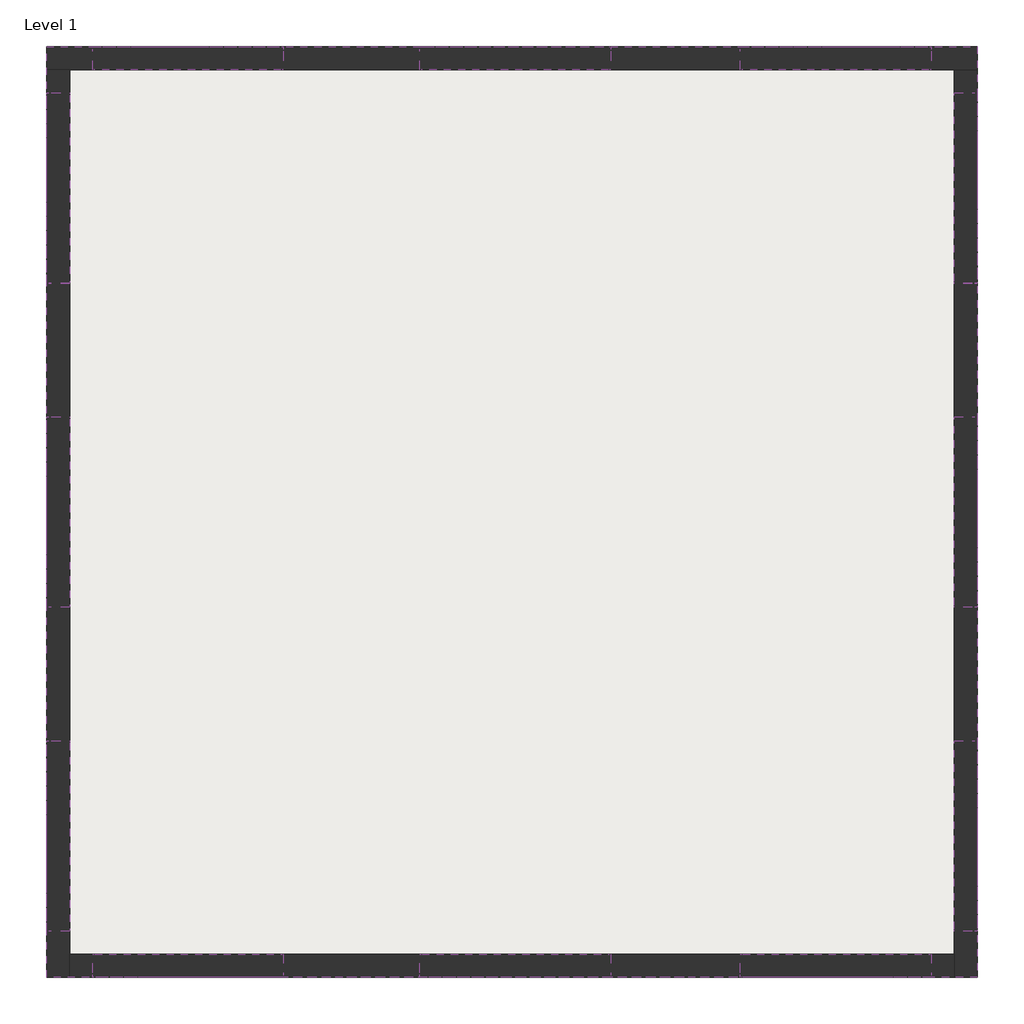
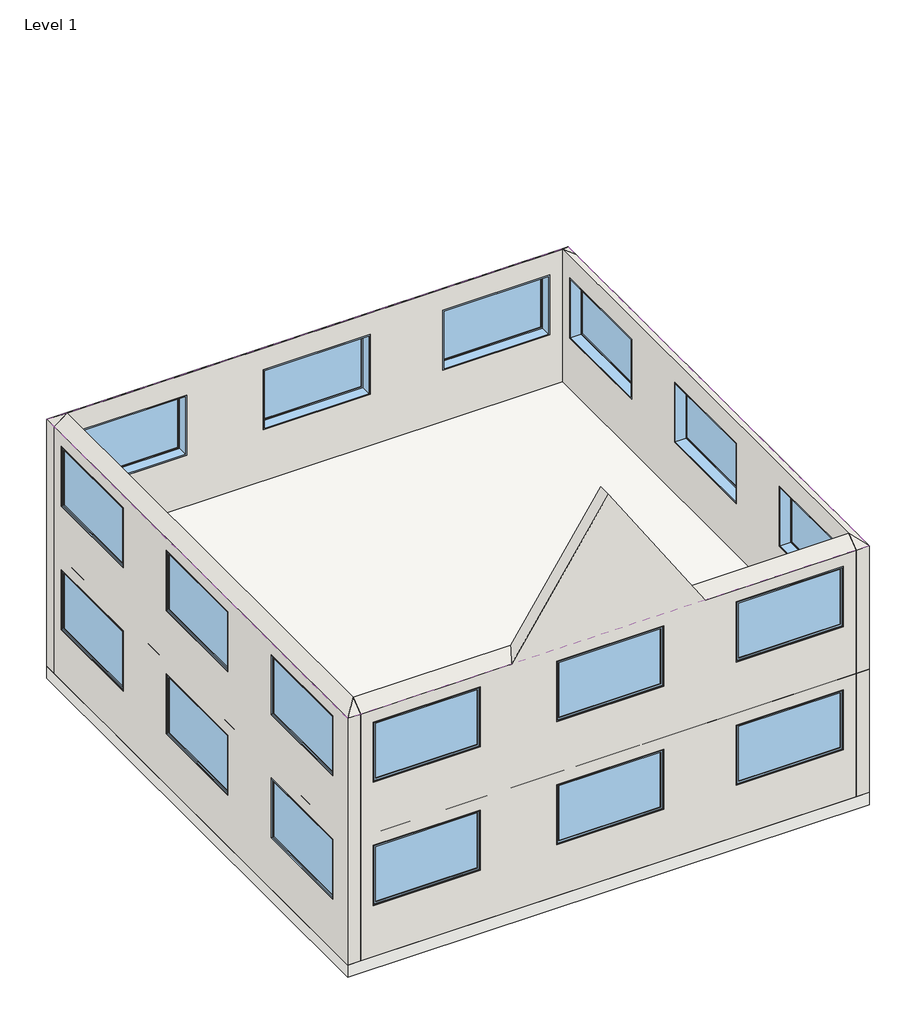
# One storey: 24 windows, 4 walls, 2 slabs, 1 roof.
"""IFC4 building model written with IfcOpenShell, lengths in millimetres."""

import ifcopenshell
import ifcopenshell.guid

model = None  # the IFC model being written
_history = None  # IfcOwnerHistory: only IFC2X3 demands one
_inside = {}  # id of a spatial element -> (the spatial element, [elements in it])
_under = {}  # id of a project, library or spatial element -> (it, [spatial elements below it])
_declared = {}  # id of a project -> (the project, [libraries it declares])
_typed = {}  # id of a type object -> (the type object, [elements of that type])
_made_of = {}  # id of a material, layer set ... -> (it, [elements and type objects made of it])


def new_model(schema):
    """Start an empty IFC model of exactly this schema.

    Asked for "IFC4X3", IfcOpenShell would pick the latest addendum, in which some entities
    have other attributes; the version numbers below select the first issue.
    IFC2X3 requires an IfcOwnerHistory on every rooted entity: one is made here for all.
    """
    global model, _history
    if schema == "IFC4X3":
        model = ifcopenshell.file(schema_version=(4, 3, 0, 0))
    else:
        model = ifcopenshell.file(schema=schema)
    _inside.clear()
    _under.clear()
    _declared.clear()
    _typed.clear()
    _made_of.clear()
    _history = None
    if model.schema == "IFC2X3":
        org = make("IfcOrganization", Name="unknown")
        user = make(
            "IfcPersonAndOrganization",
            ThePerson=make("IfcPerson", FamilyName="unknown"),
            TheOrganization=org,
        )
        app = make(
            "IfcApplication",
            ApplicationDeveloper=org,
            Version="unknown",
            ApplicationFullName="unknown",
            ApplicationIdentifier="unknown",
        )
        _history = make(
            "IfcOwnerHistory",
            OwningUser=user,
            OwningApplication=app,
            ChangeAction="ADDED",
            CreationDate=0,
        )
    return model


def make(cls, **values):
    """One entity of the class cls with the attributes given. An attribute that is None is left unset."""
    return model.create_entity(
        cls, **{name: value for name, value in values.items() if value is not None}
    )


def rooted(cls, **values):
    """An entity with a GlobalId (a new one), such as an element, a storey or a relation."""
    return make(cls, GlobalId=ifcopenshell.guid.new(), OwnerHistory=_history, **values)


def si_unit(unit_type, name, prefix=None):
    """IfcSIUnit, for example si_unit("LENGTHUNIT", "METRE", prefix="MILLI")."""
    return make("IfcSIUnit", UnitType=unit_type, Prefix=prefix, Name=name)


def assignment(units):
    """IfcUnitAssignment: the units of a project."""
    return None if units is None else make("IfcUnitAssignment", Units=units)


def point(xyz):
    """IfcCartesianPoint."""
    return None if xyz is None else make("IfcCartesianPoint", Coordinates=xyz)


def direction(xyz):
    """IfcDirection."""
    return None if xyz is None else make("IfcDirection", DirectionRatios=xyz)


def frame(location, z_axis=None, x_axis=None):
    """IfcAxis2Placement3D, a coordinate frame: its origin and axes. An axis left out is left unset."""
    return make(
        "IfcAxis2Placement3D",
        Location=point(location),
        Axis=direction(z_axis),
        RefDirection=direction(x_axis),
    )


def origin():
    """The frame at (0, 0, 0) with its axes left unset."""
    return frame((0.0, 0.0, 0.0))


def place(relative_to, where):
    """IfcLocalPlacement: puts the frame where relative to a parent placement (None: the world)."""
    return make(
        "IfcLocalPlacement", PlacementRelTo=relative_to, RelativePlacement=where
    )


def context(
    kind, dimensions, precision=None, world=None, true_north=None, identifier=None
):
    """IfcGeometricRepresentationContext, for example the 3D "Model" context."""
    return make(
        "IfcGeometricRepresentationContext",
        ContextIdentifier=identifier,
        ContextType=kind,
        CoordinateSpaceDimension=dimensions,
        Precision=precision,
        WorldCoordinateSystem=world,
        TrueNorth=true_north,
    )


def project(units=None, contexts=None):
    """IfcProject with its units and contexts."""
    return rooted(
        "IfcProject",
        Name="project",
        RepresentationContexts=contexts,
        UnitsInContext=assignment(units),
    )


def spatial(cls, under=None, at=None, **own):
    """A site, building, storey or space (cls), placed at a placement, below another one or the project."""
    s = rooted(cls, ObjectPlacement=at, **own)
    if under is not None:
        _under.setdefault(under.id(), (under, []))[1].append(s)
    return s


def polyline(points):
    """IfcPolyline through the points."""
    return make("IfcPolyline", Points=[point(p) for p in points])


def outline(outer, holes=None, kind="AREA"):
    """IfcArbitraryClosedProfileDef: a profile drawn as a closed curve; with holes, ...WithVoids."""
    if holes is None:
        return make("IfcArbitraryClosedProfileDef", ProfileType=kind, OuterCurve=outer)
    return make(
        "IfcArbitraryProfileDefWithVoids",
        ProfileType=kind,
        OuterCurve=outer,
        InnerCurves=holes,
    )


def extrude(swept, where, along, depth):
    """IfcExtrudedAreaSolid: the profile swept, set in the frame where, extruded along a direction by depth."""
    return make(
        "IfcExtrudedAreaSolid",
        SweptArea=swept,
        Position=where,
        ExtrudedDirection=direction(along),
        Depth=depth,
    )


def faces_of(points, faces, orient=None, outer=None):
    """IfcFace entities. A face is a list of loops; a loop is a list of indices into points, from 0.

    orient and outer hold one flag for each loop. By default every Orientation is true, the
    first loop of a face is its IfcFaceOuterBound and the others are IfcFaceBound.
    """
    made = []
    for i, loops in enumerate(faces):
        bounds = []
        for j, loop in enumerate(loops):
            is_outer = j == 0 if outer is None else outer[i][j]
            bounds.append(
                make(
                    "IfcFaceOuterBound" if is_outer else "IfcFaceBound",
                    Bound=make("IfcPolyLoop", Polygon=[points[k] for k in loop]),
                    Orientation=True if orient is None else orient[i][j],
                )
            )
        made.append(make("IfcFace", Bounds=bounds))
    return made


def faceted_brep(points, faces, orient=None, outer=None, voids=None):
    """IfcFacetedBrep: a solid bounded by flat faces; with voids (closed shells), ...WithVoids."""
    shared = [point(p) for p in points]
    hull = make("IfcClosedShell", CfsFaces=faces_of(shared, faces, orient, outer))
    if voids is None:
        return make("IfcFacetedBrep", Outer=hull)
    return make(
        "IfcFacetedBrepWithVoids",
        Outer=hull,
        Voids=[
            make(cls, CfsFaces=faces_of(shared, fs, o, b)) for cls, fs, o, b in voids
        ],
    )


def shape(context_of_items, identifier, shape_type, items):
    """IfcShapeRepresentation: the items that make up one representation, for example the "Body"."""
    return make(
        "IfcShapeRepresentation",
        ContextOfItems=context_of_items,
        RepresentationIdentifier=identifier,
        RepresentationType=shape_type,
        Items=items,
    )


def source(mapping_origin, context_of_items, identifier, shape_type, items):
    """IfcRepresentationMap: a shape defined once, which mapped items show again and again."""
    return make(
        "IfcRepresentationMap",
        MappingOrigin=mapping_origin,
        MappedRepresentation=shape(context_of_items, identifier, shape_type, items),
    )


def transform(
    local_origin,
    x_axis=None,
    y_axis=None,
    z_axis=None,
    scale=None,
    scale2=None,
    scale3=None,
    uniform=True,
):
    """IfcCartesianTransformationOperator3D, or its non-uniform kind. x_axis, y_axis, z_axis: its Axis1, 2, 3."""
    if uniform:
        return make(
            "IfcCartesianTransformationOperator3D",
            Axis1=direction(x_axis),
            Axis2=direction(y_axis),
            LocalOrigin=point(local_origin),
            Scale=scale,
            Axis3=direction(z_axis),
        )
    return make(
        "IfcCartesianTransformationOperator3DnonUniform",
        Axis1=direction(x_axis),
        Axis2=direction(y_axis),
        LocalOrigin=point(local_origin),
        Scale=scale,
        Axis3=direction(z_axis),
        Scale2=scale2,
        Scale3=scale3,
    )


def mapped(mapping_source, mapping_target):
    """IfcMappedItem: shows the shape of a source again, moved by a transform."""
    return make(
        "IfcMappedItem", MappingSource=mapping_source, MappingTarget=mapping_target
    )


def made_of(thing, what):
    """Note that an element or type object is made of a material, layer set ...; save() writes the relation."""
    if what is not None:
        _made_of.setdefault(what.id(), (what, []))[1].append(thing)
    return thing


def element(
    cls,
    number,
    at=None,
    inside=None,
    cuts=None,
    type_object=None,
    material=None,
    context=None,
    identifier="Body",
    shape_type=None,
    held_by="IfcProductDefinitionShape",
    body=None,
    shapes=None,
    **own,
):
    """One element of the class cls, such as IfcWall. Its Tag is "e" and its number.

    at: its placement. inside: the storey or other place that contains it. cuts: it is an
    opening in that element (IfcRelVoidsElement). A single representation is given by context,
    identifier, shape_type and body (its items); several are given by shapes. held_by: the class
    of the entity that holds the representations. save() writes the other relations.
    """
    e = rooted(cls, Tag="e%d" % number, ObjectPlacement=at, **own)
    if body is not None:
        shapes = [shape(context, identifier, shape_type, body)]
    if shapes is not None:
        e.Representation = make(held_by, Representations=shapes)
    if inside is not None:
        _inside.setdefault(inside.id(), (inside, []))[1].append(e)
    if cuts is not None:
        rooted(
            "IfcRelVoidsElement", RelatingBuildingElement=cuts, RelatedOpeningElement=e
        )
    if type_object is not None:
        _typed.setdefault(type_object.id(), (type_object, []))[1].append(e)
    return made_of(e, material)


def aggregate(whole, parts):
    """IfcRelAggregates: a whole, such as a stair, and the parts it consists of."""
    return rooted("IfcRelAggregates", RelatingObject=whole, RelatedObjects=parts)


def save(model, path):
    """Write the relations noted so far, then the file.

    IfcRelAggregates (storeys below a building ...), IfcRelContainedInSpatialStructure (elements
    in a storey), IfcRelDefinesByType, IfcRelAssociatesMaterial and IfcRelDeclares: one each for
    every whole, place, type object, material and project.
    """
    for whole, parts in _under.values():
        aggregate(whole, parts)
    for where, things in _inside.values():
        rooted(
            "IfcRelContainedInSpatialStructure",
            RelatedElements=things,
            RelatingStructure=where,
        )
    for kind, things in _typed.values():
        rooted("IfcRelDefinesByType", RelatedObjects=things, RelatingType=kind)
    for what, things in _made_of.values():
        rooted("IfcRelAssociatesMaterial", RelatedObjects=things, RelatingMaterial=what)
    for by, libraries in _declared.values():
        rooted("IfcRelDeclares", RelatingContext=by, RelatedDefinitions=libraries)
    model.write(path)


def m_fixed_2500_x_1486mm_baf7df51(model_context):
    return source(origin(), model_context, "Body", "SweptSolid", [
        extrude(outline(polyline([(-1187.0, 130.4), (1187.0, 130.4), (1187.0, 118.4), (-1187.0, 118.4), (-1187.0, 130.4)])), frame((0.0, 0.0, 978.0), z_axis=(0.0, 0.0, 1.0), x_axis=(1.0, 0.0, 0.0)), (0.0, 0.0, 1.0), 1360.5),
        extrude(outline(polyline([(2382.5, -1231.0), (934.0, -1231.0), (934.0, 1231.0), (2382.5, 1231.0), (2382.5, -1231.0)]), holes=[polyline([(2338.5, -1187.0), (2338.5, 1187.0), (978.0, 1187.0), (978.0, -1187.0), (2338.5, -1187.0)])]), frame((0.0, 102.4, 0.0), z_axis=(0.0, 1.0, 0.0), x_axis=(0.0, 0.0, 1.0)), (0.0, 0.0, 1.0), 44.0),
        extrude(outline(polyline([(2401.5, -1250.0), (915.0, -1250.0), (915.0, 1250.0), (2401.5, 1250.0), (2401.5, -1250.0)]), holes=[polyline([(2382.5, -1231.0), (2382.5, 1231.0), (934.0, 1231.0), (934.0, -1231.0), (2382.5, -1231.0)])]), frame((0.0, 102.4, 0.0), z_axis=(0.0, 1.0, 0.0), x_axis=(0.0, 0.0, 1.0)), (0.0, 0.0, 1.0), 63.0),
        extrude(outline(polyline([(2401.5, -1250.0), (915.0, -1250.0), (915.0, 1250.0), (2401.5, 1250.0), (2401.5, -1250.0)]), holes=[polyline([(2369.5, -1218.0), (2369.5, 1218.0), (947.0, 1218.0), (947.0, -1218.0), (2369.5, -1218.0)])]), frame((0.0, -139.4, 0.0), z_axis=(0.0, 1.0, 0.0), x_axis=(0.0, 0.0, 1.0)), (0.0, 0.0, 1.0), 241.8),
    ])


def m_fixed_2500_x_1486mm_49bc14c1(model_context):
    return source(origin(), model_context, "Body", "SweptSolid", [
        extrude(outline(polyline([(-1187.0, -130.4), (-1187.0, -118.4), (1187.0, -118.4), (1187.0, -130.4), (-1187.0, -130.4)])), frame((0.0, 0.0, 978.0), z_axis=(0.0, 0.0, 1.0), x_axis=(1.0, 0.0, 0.0)), (0.0, 0.0, 1.0), 1360.5),
        extrude(outline(polyline([(2382.5, -1231.0), (934.0, -1231.0), (934.0, 1231.0), (2382.5, 1231.0), (2382.5, -1231.0)]), holes=[polyline([(2338.5, -1187.0), (2338.5, 1187.0), (978.0, 1187.0), (978.0, -1187.0), (2338.5, -1187.0)])]), frame((0.0, -146.4, 0.0), z_axis=(0.0, 1.0, 0.0), x_axis=(0.0, 0.0, 1.0)), (0.0, 0.0, 1.0), 44.0),
        extrude(outline(polyline([(2401.5, -1250.0), (915.0, -1250.0), (915.0, 1250.0), (2401.5, 1250.0), (2401.5, -1250.0)]), holes=[polyline([(2382.5, -1231.0), (2382.5, 1231.0), (934.0, 1231.0), (934.0, -1231.0), (2382.5, -1231.0)])]), frame((0.0, -165.4, 0.0), z_axis=(0.0, 1.0, 0.0), x_axis=(0.0, 0.0, 1.0)), (0.0, 0.0, 1.0), 63.0),
        extrude(outline(polyline([(2401.5, -1250.0), (915.0, -1250.0), (915.0, 1250.0), (2401.5, 1250.0), (2401.5, -1250.0)]), holes=[polyline([(2369.5, -1218.0), (2369.5, 1218.0), (947.0, 1218.0), (947.0, -1218.0), (2369.5, -1218.0)])]), frame((0.0, -102.4, 0.0), z_axis=(0.0, 1.0, 0.0), x_axis=(0.0, 0.0, 1.0)), (0.0, 0.0, 1.0), 241.8),
    ])


model = new_model("IFC4")

# Units and contexts
model_context = context("Model", 3, world=origin())
ifc_project = project(units=[si_unit("LENGTHUNIT", "METRE", prefix="MILLI")], contexts=[model_context])

# Site, building, storey
site = spatial("IfcSite", under=ifc_project)
building = spatial("IfcBuilding", under=site)
storey = spatial("IfcBuildingStorey", under=building, Name="Level 1", Elevation=0.0)

# Roof
placement = place(None, origin())
element("IfcRoof", 1, ObjectType="Generic Roof - 300mm", at=placement, inside=storey, context=model_context, shape_type="Brep", body=[
    faceted_brep([(21465.644102, 9062.7173115, 6096.0), (15369.644102, 2966.7173115, 10668.0170156), (9273.644102, 9062.7173115, 6096.0), (9273.644102, -3129.2826885, 6096.0), (13109.1679245, -3129.2826885, 6096.0), (12998.044102, -3129.2826885, 6096.0), (21465.644102, -3129.2826885, 6096.0), (17741.244102, -3129.2826885, 6096.0), (17630.1202795, -3129.2826885, 6096.0), (15369.644102, 1410.2073073, 9500.6301678), (15369.644102, -3129.2826885, 9500.6301678), (21465.644102, 9062.7173115, 6471.0005024), (9273.644102, 9062.7173115, 6471.0005024), (15369.644102, 2966.7173115, 11043.0175181), (9273.644102, -3129.2826885, 6471.0005024), (12998.044102, -3129.2826885, 6471.0005024), (15369.644102, 1633.366253, 10043.0005024), (17741.244102, -3129.2826885, 6471.0005024), (21465.644102, -3129.2826885, 6471.0005024), (15369.644102, -3129.2826885, 10043.0005024)], [[[0, 1, 2]], [[2, 1, 3]], [[4, 5, 3, 1, 6, 7, 8, 9]], [[6, 1, 0]], [[4, 9, 10]], [[8, 10, 9]], [[11, 12, 13]], [[12, 14, 13]], [[15, 16, 17, 18, 13, 14]], [[18, 11, 13]], [[15, 19, 16]], [[17, 16, 19]], [[6, 18, 17, 7]], [[0, 11, 18, 6]], [[2, 12, 11, 0]], [[3, 14, 12, 2]], [[5, 15, 14, 3]], [[17, 19, 15, 5, 4, 10, 8, 7]]]),
])

# Slabs
element("IfcSlab", 2, ObjectType="Generic Floor - 304.8mm", at=placement, inside=storey, context=model_context, shape_type="Brep", body=[
    faceted_brep([(21465.644102, 9062.7173115, -304.8), (21465.644102, -3129.2826885, -304.8), (9273.644102, -3129.2826885, -304.8), (9273.644102, 9062.7173115, -304.8), (21465.644102, 9062.7173115, 0.0), (9273.644102, 9062.7173115, 0.0), (9273.644102, -3129.2826885, 0.0), (9578.444102, -3129.2826885, 0.0), (21160.844102, -3129.2826885, 0.0), (21465.644102, -3129.2826885, 0.0), (21465.644102, 8757.9173115, 0.0)], [[[0, 1, 2, 3]], [[4, 5, 6, 7, 8, 9, 10]], [[1, 0, 4, 10, 9]], [[2, 1, 9, 8, 7, 6]], [[3, 2, 6, 5]], [[0, 3, 5, 4]]]),
])
element("IfcSlab", 3, ObjectType="Generic Floor - 304.8mm", at=placement, inside=storey, context=model_context, shape_type="SweptSolid", body=[
    extrude(outline(polyline([(21465.644102, 9062.7173115), (21465.644102, -3129.2826885), (9273.644102, -3129.2826885), (9273.644102, 9062.7173115), (21465.644102, 9062.7173115)])), frame((0.0, 0.0, 2743.2), z_axis=(0.0, 0.0, 1.0), x_axis=(1.0, 0.0, 0.0)), (0.0, 0.0, 1.0), 304.8),
])

# Walls
element("IfcWall", 4, ObjectType="Generic - 304.8mm", at=placement, inside=storey, context=model_context, shape_type="Brep", body=[
    faceted_brep([(9273.644102, 8757.9173115, 0.0), (9578.444102, 8757.9173115, 0.0), (21160.844102, 8757.9173115, 0.0), (21465.644102, 8757.9173115, 0.0), (21465.644102, 8757.9173115, 6096.0), (21160.844102, 8757.9173115, 6324.6008508), (9578.444102, 8757.9173115, 6324.6008508), (9273.644102, 8757.9173115, 6096.0), (14163.244102, 8757.9173115, 4309.5), (14163.244102, 8757.9173115, 5796.0), (16663.244102, 8757.9173115, 5796.0), (16663.244102, 8757.9173115, 4309.5), (9876.044102, 8757.9173115, 4309.5), (9876.044102, 8757.9173115, 5796.0), (12376.044102, 8757.9173115, 5796.0), (12376.044102, 8757.9173115, 4309.5), (18363.244102, 8757.9173115, 4309.5), (18363.244102, 8757.9173115, 5796.0), (20863.244102, 8757.9173115, 5796.0), (20863.244102, 8757.9173115, 4309.5), (18363.244102, 8757.9173115, 1261.5), (18363.244102, 8757.9173115, 2748.0), (20863.244102, 8757.9173115, 2748.0), (20863.244102, 8757.9173115, 1261.5), (9876.044102, 8757.9173115, 1261.5), (9876.044102, 8757.9173115, 2748.0), (12376.044102, 8757.9173115, 2748.0), (12376.044102, 8757.9173115, 1261.5), (14163.244102, 8757.9173115, 1261.5), (14163.244102, 8757.9173115, 2748.0), (16663.244102, 8757.9173115, 2748.0), (16663.244102, 8757.9173115, 1261.5), (9273.644102, 9062.7173115, 0.0), (9273.644102, 9062.7173115, 6096.0), (21465.644102, 9062.7173115, 6096.0), (21465.644102, 9062.7173115, 0.0), (14163.244102, 9062.7173115, 4309.5), (16663.244102, 9062.7173115, 4309.5), (16663.244102, 9062.7173115, 5796.0), (14163.244102, 9062.7173115, 5796.0), (9876.044102, 9062.7173115, 4309.5), (12376.044102, 9062.7173115, 4309.5), (12376.044102, 9062.7173115, 5796.0), (9876.044102, 9062.7173115, 5796.0), (18363.244102, 9062.7173115, 4309.5), (20863.244102, 9062.7173115, 4309.5), (20863.244102, 9062.7173115, 5796.0), (18363.244102, 9062.7173115, 5796.0), (18363.244102, 9062.7173115, 1261.5), (20863.244102, 9062.7173115, 1261.5), (20863.244102, 9062.7173115, 2748.0), (18363.244102, 9062.7173115, 2748.0), (9876.044102, 9062.7173115, 1261.5), (12376.044102, 9062.7173115, 1261.5), (12376.044102, 9062.7173115, 2748.0), (9876.044102, 9062.7173115, 2748.0), (14163.244102, 9062.7173115, 1261.5), (16663.244102, 9062.7173115, 1261.5), (16663.244102, 9062.7173115, 2748.0), (14163.244102, 9062.7173115, 2748.0)], [[[0, 1, 2, 3, 4, 5, 6, 7], [8, 9, 10, 11], [12, 13, 14, 15], [16, 17, 18, 19], [20, 21, 22, 23], [24, 25, 26, 27], [28, 29, 30, 31]], [[32, 33, 34, 35], [36, 37, 38, 39], [40, 41, 42, 43], [44, 45, 46, 47], [48, 49, 50, 51], [52, 53, 54, 55], [56, 57, 58, 59]], [[3, 2, 1, 0, 32, 35]], [[4, 3, 35, 34]], [[0, 7, 33, 32]], [[9, 8, 36, 39]], [[10, 9, 39, 38]], [[11, 10, 38, 37]], [[8, 11, 37, 36]], [[13, 12, 40, 43]], [[14, 13, 43, 42]], [[15, 14, 42, 41]], [[12, 15, 41, 40]], [[17, 16, 44, 47]], [[18, 17, 47, 46]], [[19, 18, 46, 45]], [[16, 19, 45, 44]], [[21, 20, 48, 51]], [[22, 21, 51, 50]], [[23, 22, 50, 49]], [[20, 23, 49, 48]], [[25, 24, 52, 55]], [[26, 25, 55, 54]], [[27, 26, 54, 53]], [[24, 27, 53, 52]], [[29, 28, 56, 59]], [[30, 29, 59, 58]], [[31, 30, 58, 57]], [[28, 31, 57, 56]], [[7, 6, 33]], [[6, 5, 34, 33]], [[5, 4, 34]]]),
])
element("IfcWall", 5, ObjectType="Generic - 304.8mm", at=placement, inside=storey, context=model_context, shape_type="Brep", body=[
    faceted_brep([(21160.844102, 8757.9173115, 0.0), (21160.844102, -2824.4826885, 0.0), (21160.844102, -3129.2826885, 0.0), (21160.844102, -3129.2826885, 6096.0), (21160.844102, -2824.4826885, 6324.6008508), (21160.844102, 8757.9173115, 6324.6008508), (21160.844102, -26.8826885, 4309.5), (21160.844102, -26.8826885, 5796.0), (21160.844102, -2526.8826885, 5796.0), (21160.844102, -2526.8826885, 4309.5), (21160.844102, 8460.3173115, 4309.5), (21160.844102, 8460.3173115, 5796.0), (21160.844102, 5960.3173115, 5796.0), (21160.844102, 5960.3173115, 4309.5), (21160.844102, 4216.7173115, 4309.5), (21160.844102, 4216.7173115, 5796.0), (21160.844102, 1716.7173115, 5796.0), (21160.844102, 1716.7173115, 4309.5), (21160.844102, 4216.7173115, 1261.5), (21160.844102, 4216.7173115, 2748.0), (21160.844102, 1716.7173115, 2748.0), (21160.844102, 1716.7173115, 1261.5), (21160.844102, 8460.3173115, 1261.5), (21160.844102, 8460.3173115, 2748.0), (21160.844102, 5960.3173115, 2748.0), (21160.844102, 5960.3173115, 1261.5), (21160.844102, -26.8826885, 1261.5), (21160.844102, -26.8826885, 2748.0), (21160.844102, -2526.8826885, 2748.0), (21160.844102, -2526.8826885, 1261.5), (21465.644102, 8757.9173115, 0.0), (21465.644102, 8757.9173115, 6096.0), (21465.644102, -3129.2826885, 6096.0), (21465.644102, -3129.2826885, 0.0), (21465.644102, -26.8826885, 4309.5), (21465.644102, -2526.8826885, 4309.5), (21465.644102, -2526.8826885, 5796.0), (21465.644102, -26.8826885, 5796.0), (21465.644102, 8460.3173115, 4309.5), (21465.644102, 5960.3173115, 4309.5), (21465.644102, 5960.3173115, 5796.0), (21465.644102, 8460.3173115, 5796.0), (21465.644102, 4216.7173115, 4309.5), (21465.644102, 1716.7173115, 4309.5), (21465.644102, 1716.7173115, 5796.0), (21465.644102, 4216.7173115, 5796.0), (21465.644102, 4216.7173115, 1261.5), (21465.644102, 1716.7173115, 1261.5), (21465.644102, 1716.7173115, 2748.0), (21465.644102, 4216.7173115, 2748.0), (21465.644102, 8460.3173115, 1261.5), (21465.644102, 5960.3173115, 1261.5), (21465.644102, 5960.3173115, 2748.0), (21465.644102, 8460.3173115, 2748.0), (21465.644102, -26.8826885, 1261.5), (21465.644102, -2526.8826885, 1261.5), (21465.644102, -2526.8826885, 2748.0), (21465.644102, -26.8826885, 2748.0)], [[[0, 1, 2, 3, 4, 5], [6, 7, 8, 9], [10, 11, 12, 13], [14, 15, 16, 17], [18, 19, 20, 21], [22, 23, 24, 25], [26, 27, 28, 29]], [[30, 31, 32, 33], [34, 35, 36, 37], [38, 39, 40, 41], [42, 43, 44, 45], [46, 47, 48, 49], [50, 51, 52, 53], [54, 55, 56, 57]], [[2, 1, 0, 30, 33]], [[0, 5, 31, 30]], [[3, 2, 33, 32]], [[7, 6, 34, 37]], [[8, 7, 37, 36]], [[9, 8, 36, 35]], [[6, 9, 35, 34]], [[11, 10, 38, 41]], [[12, 11, 41, 40]], [[13, 12, 40, 39]], [[10, 13, 39, 38]], [[15, 14, 42, 45]], [[16, 15, 45, 44]], [[17, 16, 44, 43]], [[14, 17, 43, 42]], [[19, 18, 46, 49]], [[20, 19, 49, 48]], [[21, 20, 48, 47]], [[18, 21, 47, 46]], [[23, 22, 50, 53]], [[24, 23, 53, 52]], [[25, 24, 52, 51]], [[22, 25, 51, 50]], [[27, 26, 54, 57]], [[28, 27, 57, 56]], [[29, 28, 56, 55]], [[26, 29, 55, 54]], [[5, 4, 32, 31]], [[4, 3, 32]]]),
])
element("IfcWall", 6, ObjectType="Generic - 304.8mm", at=placement, inside=storey, context=model_context, shape_type="Brep", body=[
    faceted_brep([(9578.444102, -3129.2826885, 0.0), (9578.444102, -2824.4826885, 0.0), (9578.444102, 8757.9173115, 0.0), (9578.444102, 8757.9173115, 6324.6008508), (9578.444102, -2824.4826885, 6324.6008508), (9578.444102, -3129.2826885, 6096.0), (9578.444102, 1716.7173115, 4309.5), (9578.444102, 1716.7173115, 5796.0), (9578.444102, 4216.7173115, 5796.0), (9578.444102, 4216.7173115, 4309.5), (9578.444102, 5960.3173115, 4309.5), (9578.444102, 5960.3173115, 5796.0), (9578.444102, 8460.3173115, 5796.0), (9578.444102, 8460.3173115, 4309.5), (9578.444102, -2526.8826885, 4309.5), (9578.444102, -2526.8826885, 5796.0), (9578.444102, -26.8826885, 5796.0), (9578.444102, -26.8826885, 4309.5), (9578.444102, -2526.8826885, 1261.5), (9578.444102, -2526.8826885, 2748.0), (9578.444102, -26.8826885, 2748.0), (9578.444102, -26.8826885, 1261.5), (9578.444102, 5960.3173115, 1261.5), (9578.444102, 5960.3173115, 2748.0), (9578.444102, 8460.3173115, 2748.0), (9578.444102, 8460.3173115, 1261.5), (9578.444102, 1716.7173115, 1261.5), (9578.444102, 1716.7173115, 2748.0), (9578.444102, 4216.7173115, 2748.0), (9578.444102, 4216.7173115, 1261.5), (9273.644102, -3129.2826885, 0.0), (9273.644102, -3129.2826885, 6096.0), (9273.644102, 8757.9173115, 6096.0), (9273.644102, 8757.9173115, 0.0), (9273.644102, 1716.7173115, 4309.5), (9273.644102, 4216.7173115, 4309.5), (9273.644102, 4216.7173115, 5796.0), (9273.644102, 1716.7173115, 5796.0), (9273.644102, 5960.3173115, 4309.5), (9273.644102, 8460.3173115, 4309.5), (9273.644102, 8460.3173115, 5796.0), (9273.644102, 5960.3173115, 5796.0), (9273.644102, -2526.8826885, 4309.5), (9273.644102, -26.8826885, 4309.5), (9273.644102, -26.8826885, 5796.0), (9273.644102, -2526.8826885, 5796.0), (9273.644102, -2526.8826885, 1261.5), (9273.644102, -26.8826885, 1261.5), (9273.644102, -26.8826885, 2748.0), (9273.644102, -2526.8826885, 2748.0), (9273.644102, 5960.3173115, 1261.5), (9273.644102, 8460.3173115, 1261.5), (9273.644102, 8460.3173115, 2748.0), (9273.644102, 5960.3173115, 2748.0), (9273.644102, 1716.7173115, 1261.5), (9273.644102, 4216.7173115, 1261.5), (9273.644102, 4216.7173115, 2748.0), (9273.644102, 1716.7173115, 2748.0)], [[[0, 1, 2, 3, 4, 5], [6, 7, 8, 9], [10, 11, 12, 13], [14, 15, 16, 17], [18, 19, 20, 21], [22, 23, 24, 25], [26, 27, 28, 29]], [[30, 31, 32, 33], [34, 35, 36, 37], [38, 39, 40, 41], [42, 43, 44, 45], [46, 47, 48, 49], [50, 51, 52, 53], [54, 55, 56, 57]], [[2, 1, 0, 30, 33]], [[3, 2, 33, 32]], [[0, 5, 31, 30]], [[7, 6, 34, 37]], [[8, 7, 37, 36]], [[9, 8, 36, 35]], [[6, 9, 35, 34]], [[11, 10, 38, 41]], [[12, 11, 41, 40]], [[13, 12, 40, 39]], [[10, 13, 39, 38]], [[15, 14, 42, 45]], [[16, 15, 45, 44]], [[17, 16, 44, 43]], [[14, 17, 43, 42]], [[19, 18, 46, 49]], [[20, 19, 49, 48]], [[21, 20, 48, 47]], [[18, 21, 47, 46]], [[23, 22, 50, 53]], [[24, 23, 53, 52]], [[25, 24, 52, 51]], [[22, 25, 51, 50]], [[27, 26, 54, 57]], [[28, 27, 57, 56]], [[29, 28, 56, 55]], [[26, 29, 55, 54]], [[5, 4, 31]], [[4, 3, 32, 31]]]),
])
element("IfcWall", 7, ObjectType="Generic - 304.8mm", at=placement, inside=storey, context=model_context, shape_type="Brep", body=[
    faceted_brep([(9578.444102, -3129.2826885, 0.0), (21160.844102, -3129.2826885, 0.0), (21160.844102, -3129.2826885, 6096.0), (17741.244102, -3129.2826885, 6096.0), (17630.1202795, -3129.2826885, 6096.0), (15369.644102, -3129.2826885, 9500.6301678), (13109.1679245, -3129.2826885, 6096.0), (12998.044102, -3129.2826885, 6096.0), (9578.444102, -3129.2826885, 6096.0), (14163.244102, -3129.2826885, 4309.5), (14163.244102, -3129.2826885, 5796.0), (16663.244102, -3129.2826885, 5796.0), (16663.244102, -3129.2826885, 4309.5), (9876.044102, -3129.2826885, 4309.5), (9876.044102, -3129.2826885, 5796.0), (12376.044102, -3129.2826885, 5796.0), (12376.044102, -3129.2826885, 4309.5), (18363.244102, -3129.2826885, 4309.5), (18363.244102, -3129.2826885, 5796.0), (20863.244102, -3129.2826885, 5796.0), (20863.244102, -3129.2826885, 4309.5), (18363.244102, -3129.2826885, 1261.5), (18363.244102, -3129.2826885, 2748.0), (20863.244102, -3129.2826885, 2748.0), (20863.244102, -3129.2826885, 1261.5), (9876.044102, -3129.2826885, 1261.5), (9876.044102, -3129.2826885, 2748.0), (12376.044102, -3129.2826885, 2748.0), (12376.044102, -3129.2826885, 1261.5), (14163.244102, -3129.2826885, 1261.5), (14163.244102, -3129.2826885, 2748.0), (16663.244102, -3129.2826885, 2748.0), (16663.244102, -3129.2826885, 1261.5), (9578.444102, -2824.4826885, 0.0), (9578.444102, -2824.4826885, 6324.6008508), (13260.9455778, -2824.4826885, 6324.6008508), (15369.644102, -2824.4826885, 9500.6301678), (17478.3426261, -2824.4826885, 6324.6008508), (21160.844102, -2824.4826885, 6324.6008508), (21160.844102, -2824.4826885, 0.0), (14163.244102, -2824.4826885, 4309.5), (16663.244102, -2824.4826885, 4309.5), (16663.244102, -2824.4826885, 5796.0), (14163.244102, -2824.4826885, 5796.0), (9876.044102, -2824.4826885, 4309.5), (12376.044102, -2824.4826885, 4309.5), (12376.044102, -2824.4826885, 5796.0), (9876.044102, -2824.4826885, 5796.0), (18363.244102, -2824.4826885, 4309.5), (20863.244102, -2824.4826885, 4309.5), (20863.244102, -2824.4826885, 5796.0), (18363.244102, -2824.4826885, 5796.0), (18363.244102, -2824.4826885, 1261.5), (20863.244102, -2824.4826885, 1261.5), (20863.244102, -2824.4826885, 2748.0), (18363.244102, -2824.4826885, 2748.0), (9876.044102, -2824.4826885, 1261.5), (12376.044102, -2824.4826885, 1261.5), (12376.044102, -2824.4826885, 2748.0), (9876.044102, -2824.4826885, 2748.0), (14163.244102, -2824.4826885, 1261.5), (16663.244102, -2824.4826885, 1261.5), (16663.244102, -2824.4826885, 2748.0), (14163.244102, -2824.4826885, 2748.0)], [[[0, 1, 2, 3, 4, 5, 6, 7, 8], [9, 10, 11, 12], [13, 14, 15, 16], [17, 18, 19, 20], [21, 22, 23, 24], [25, 26, 27, 28], [29, 30, 31, 32]], [[33, 34, 35, 36, 37, 38, 39], [40, 41, 42, 43], [44, 45, 46, 47], [48, 49, 50, 51], [52, 53, 54, 55], [56, 57, 58, 59], [60, 61, 62, 63]], [[10, 9, 40, 43]], [[11, 10, 43, 42]], [[12, 11, 42, 41]], [[9, 12, 41, 40]], [[14, 13, 44, 47]], [[15, 14, 47, 46]], [[16, 15, 46, 45]], [[13, 16, 45, 44]], [[18, 17, 48, 51]], [[19, 18, 51, 50]], [[20, 19, 50, 49]], [[17, 20, 49, 48]], [[22, 21, 52, 55]], [[23, 22, 55, 54]], [[24, 23, 54, 53]], [[21, 24, 53, 52]], [[26, 25, 56, 59]], [[27, 26, 59, 58]], [[28, 27, 58, 57]], [[25, 28, 57, 56]], [[30, 29, 60, 63]], [[31, 30, 63, 62]], [[32, 31, 62, 61]], [[29, 32, 61, 60]], [[2, 1, 39, 38]], [[0, 8, 34, 33]], [[1, 0, 33, 39]], [[8, 7, 6, 35, 34]], [[6, 5, 36, 35]], [[5, 4, 37, 36]], [[4, 3, 2, 38, 37]]]),
])

# Windows
m_fixed_2500_x_1486mm_shape = m_fixed_2500_x_1486mm_baf7df51(model_context)
element("IfcWindow", 8, ObjectType="M_Fixed : 2500 x 1486mm", at=placement, inside=storey, context=model_context, shape_type="MappedRepresentation", body=[
    mapped(m_fixed_2500_x_1486mm_shape, transform((15413.244102, 8897.3173115, 3394.5), x_axis=(1.0, 0.0, 0.0), y_axis=(0.0, 1.0, 0.0), z_axis=(0.0, 0.0, 1.0))),
])
element("IfcWindow", 9, ObjectType="M_Fixed : 2500 x 1486mm", at=placement, inside=storey, context=model_context, shape_type="MappedRepresentation", body=[
    mapped(m_fixed_2500_x_1486mm_shape, transform((11126.044102, 8897.3173115, 3394.5), x_axis=(1.0, 0.0, 0.0), y_axis=(0.0, 1.0, 0.0), z_axis=(0.0, 0.0, 1.0))),
])
element("IfcWindow", 10, ObjectType="M_Fixed : 2500 x 1486mm", at=placement, inside=storey, context=model_context, shape_type="MappedRepresentation", body=[
    mapped(m_fixed_2500_x_1486mm_shape, transform((19613.244102, 8897.3173115, 3394.5), x_axis=(1.0, 0.0, 0.0), y_axis=(0.0, 1.0, 0.0), z_axis=(0.0, 0.0, 1.0))),
])
element("IfcWindow", 11, ObjectType="M_Fixed : 2500 x 1486mm", at=placement, inside=storey, context=model_context, shape_type="MappedRepresentation", body=[
    mapped(m_fixed_2500_x_1486mm_shape, transform((15413.244102, 8897.3173115, 346.5), x_axis=(1.0, 0.0, 0.0), y_axis=(0.0, 1.0, 0.0), z_axis=(0.0, 0.0, 1.0))),
])
element("IfcWindow", 12, ObjectType="M_Fixed : 2500 x 1486mm", at=placement, inside=storey, context=model_context, shape_type="MappedRepresentation", body=[
    mapped(m_fixed_2500_x_1486mm_shape, transform((11126.044102, 8897.3173115, 346.5), x_axis=(1.0, 0.0, 0.0), y_axis=(0.0, 1.0, 0.0), z_axis=(0.0, 0.0, 1.0))),
])
element("IfcWindow", 13, ObjectType="M_Fixed : 2500 x 1486mm", at=placement, inside=storey, context=model_context, shape_type="MappedRepresentation", body=[
    mapped(m_fixed_2500_x_1486mm_shape, transform((19613.244102, 8897.3173115, 346.5), x_axis=(1.0, 0.0, 0.0), y_axis=(0.0, 1.0, 0.0), z_axis=(0.0, 0.0, 1.0))),
])
element("IfcWindow", 14, ObjectType="M_Fixed : 2500 x 1486mm", at=placement, inside=storey, context=model_context, shape_type="MappedRepresentation", body=[
    mapped(m_fixed_2500_x_1486mm_shape, transform((21300.244102, -1276.8826885, 3394.5), x_axis=(0.0, -1.0, 0.0), y_axis=(1.0, 0.0, 0.0), z_axis=(0.0, 0.0, 1.0))),
])
element("IfcWindow", 15, ObjectType="M_Fixed : 2500 x 1486mm", at=placement, inside=storey, context=model_context, shape_type="MappedRepresentation", body=[
    mapped(m_fixed_2500_x_1486mm_shape, transform((21300.244102, 7210.3173115, 3394.5), x_axis=(0.0, -1.0, 0.0), y_axis=(1.0, 0.0, 0.0), z_axis=(0.0, 0.0, 1.0))),
])
element("IfcWindow", 16, ObjectType="M_Fixed : 2500 x 1486mm", at=placement, inside=storey, context=model_context, shape_type="MappedRepresentation", body=[
    mapped(m_fixed_2500_x_1486mm_shape, transform((21300.244102, 2966.7173115, 3394.5), x_axis=(0.0, -1.0, 0.0), y_axis=(1.0, 0.0, 0.0), z_axis=(0.0, 0.0, 1.0))),
])
element("IfcWindow", 17, ObjectType="M_Fixed : 2500 x 1486mm", at=placement, inside=storey, context=model_context, shape_type="MappedRepresentation", body=[
    mapped(m_fixed_2500_x_1486mm_shape, transform((21300.244102, -1276.8826885, 346.5), x_axis=(0.0, -1.0, 0.0), y_axis=(1.0, 0.0, 0.0), z_axis=(0.0, 0.0, 1.0))),
])
element("IfcWindow", 18, ObjectType="M_Fixed : 2500 x 1486mm", at=placement, inside=storey, context=model_context, shape_type="MappedRepresentation", body=[
    mapped(m_fixed_2500_x_1486mm_shape, transform((21300.244102, 7210.3173115, 346.5), x_axis=(0.0, -1.0, 0.0), y_axis=(1.0, 0.0, 0.0), z_axis=(0.0, 0.0, 1.0))),
])
element("IfcWindow", 19, ObjectType="M_Fixed : 2500 x 1486mm", at=placement, inside=storey, context=model_context, shape_type="MappedRepresentation", body=[
    mapped(m_fixed_2500_x_1486mm_shape, transform((21300.244102, 2966.7173115, 346.5), x_axis=(0.0, -1.0, 0.0), y_axis=(1.0, 0.0, 0.0), z_axis=(0.0, 0.0, 1.0))),
])
element("IfcWindow", 20, ObjectType="M_Fixed : 2500 x 1486mm", at=placement, inside=storey, context=model_context, shape_type="MappedRepresentation", body=[
    mapped(m_fixed_2500_x_1486mm_shape, transform((9439.044102, 2966.7173115, 3394.5), x_axis=(0.0, 1.0, 0.0), y_axis=(-1.0, 0.0, 0.0), z_axis=(0.0, 0.0, 1.0))),
])
element("IfcWindow", 21, ObjectType="M_Fixed : 2500 x 1486mm", at=placement, inside=storey, context=model_context, shape_type="MappedRepresentation", body=[
    mapped(m_fixed_2500_x_1486mm_shape, transform((9439.044102, 7210.3173115, 3394.5), x_axis=(0.0, 1.0, 0.0), y_axis=(-1.0, 0.0, 0.0), z_axis=(0.0, 0.0, 1.0))),
])
element("IfcWindow", 22, ObjectType="M_Fixed : 2500 x 1486mm", at=placement, inside=storey, context=model_context, shape_type="MappedRepresentation", body=[
    mapped(m_fixed_2500_x_1486mm_shape, transform((9439.044102, -1276.8826885, 3394.5), x_axis=(0.0, 1.0, 0.0), y_axis=(-1.0, 0.0, 0.0), z_axis=(0.0, 0.0, 1.0))),
])
element("IfcWindow", 23, ObjectType="M_Fixed : 2500 x 1486mm", at=placement, inside=storey, context=model_context, shape_type="MappedRepresentation", body=[
    mapped(m_fixed_2500_x_1486mm_shape, transform((9439.044102, 2966.7173115, 346.5), x_axis=(0.0, 1.0, 0.0), y_axis=(-1.0, 0.0, 0.0), z_axis=(0.0, 0.0, 1.0))),
])
element("IfcWindow", 24, ObjectType="M_Fixed : 2500 x 1486mm", at=placement, inside=storey, context=model_context, shape_type="MappedRepresentation", body=[
    mapped(m_fixed_2500_x_1486mm_shape, transform((9439.044102, 7210.3173115, 346.5), x_axis=(0.0, 1.0, 0.0), y_axis=(-1.0, 0.0, 0.0), z_axis=(0.0, 0.0, 1.0))),
])
element("IfcWindow", 25, ObjectType="M_Fixed : 2500 x 1486mm", at=placement, inside=storey, context=model_context, shape_type="MappedRepresentation", body=[
    mapped(m_fixed_2500_x_1486mm_shape, transform((9439.044102, -1276.8826885, 346.5), x_axis=(0.0, 1.0, 0.0), y_axis=(-1.0, 0.0, 0.0), z_axis=(0.0, 0.0, 1.0))),
])
m_fixed_2500_x_1486mm_2_shape = m_fixed_2500_x_1486mm_49bc14c1(model_context)
element("IfcWindow", 26, ObjectType="M_Fixed : 2500 x 1486mm", at=placement, inside=storey, context=model_context, shape_type="MappedRepresentation", body=[
    mapped(m_fixed_2500_x_1486mm_2_shape, transform((15413.244102, -2963.8826885, 3394.5), x_axis=(1.0, 0.0, 0.0), y_axis=(0.0, 1.0, 0.0), z_axis=(0.0, 0.0, 1.0))),
])
element("IfcWindow", 27, ObjectType="M_Fixed : 2500 x 1486mm", at=placement, inside=storey, context=model_context, shape_type="MappedRepresentation", body=[
    mapped(m_fixed_2500_x_1486mm_2_shape, transform((11126.044102, -2963.8826885, 3394.5), x_axis=(1.0, 0.0, 0.0), y_axis=(0.0, 1.0, 0.0), z_axis=(0.0, 0.0, 1.0))),
])
element("IfcWindow", 28, ObjectType="M_Fixed : 2500 x 1486mm", at=placement, inside=storey, context=model_context, shape_type="MappedRepresentation", body=[
    mapped(m_fixed_2500_x_1486mm_2_shape, transform((19613.244102, -2963.8826885, 3394.5), x_axis=(1.0, 0.0, 0.0), y_axis=(0.0, 1.0, 0.0), z_axis=(0.0, 0.0, 1.0))),
])
element("IfcWindow", 29, ObjectType="M_Fixed : 2500 x 1486mm", at=placement, inside=storey, context=model_context, shape_type="MappedRepresentation", body=[
    mapped(m_fixed_2500_x_1486mm_2_shape, transform((15413.244102, -2963.8826885, 346.5), x_axis=(1.0, 0.0, 0.0), y_axis=(0.0, 1.0, 0.0), z_axis=(0.0, 0.0, 1.0))),
])
element("IfcWindow", 30, ObjectType="M_Fixed : 2500 x 1486mm", at=placement, inside=storey, context=model_context, shape_type="MappedRepresentation", body=[
    mapped(m_fixed_2500_x_1486mm_2_shape, transform((11126.044102, -2963.8826885, 346.5), x_axis=(1.0, 0.0, 0.0), y_axis=(0.0, 1.0, 0.0), z_axis=(0.0, 0.0, 1.0))),
])
element("IfcWindow", 31, ObjectType="M_Fixed : 2500 x 1486mm", at=placement, inside=storey, context=model_context, shape_type="MappedRepresentation", body=[
    mapped(m_fixed_2500_x_1486mm_2_shape, transform((19613.244102, -2963.8826885, 346.5), x_axis=(1.0, 0.0, 0.0), y_axis=(0.0, 1.0, 0.0), z_axis=(0.0, 0.0, 1.0))),
])

save(model, "model.ifc")

# Revit data of these elements
# Project information
#   Project Issue Date = "Issue Date"
#   Project Status = "Project Status"
#   Client Name = "Owner"
#   Project Address = "Enter address here"
#   Project Name = "Project Name"
#   Project Number = "Project Number"
# Type "Generic Roof - 300mm"
#   Layers, outside or top first: 300 mm no material (function 1)
# Type "Generic Floor - 304.8mm"
#   Function = 0
#   Layers, outside or top first: 304.8 mm no material (function 1)
# Type "Generic - 304.8mm"
#   Layers, outside or top first: 304.8 mm no material (function 1)
# Type "M_Fixed : 2500 x 1486mm"
#   Type Mark = "19"
#   Height = 1486.5 mm
#   Default Sill Height = 915 mm
#   Width = 2500 mm
#   Window Inset = 19 mm
#   Frame Exterior Material = Sash
#   Frame Interior Material = Sash
#   Glass Pane Material = Glass
#   Sash = Sash
#   Wall Closure = (empty or 0)
# Element 1 (IfcRoof, "Generic Roof - 300mm")
#   built-in parameter 1001705 = 36.2304 (stored number, unit not read)
#   built-in parameter 1001701 = 20 (stored number, unit not read)
#   built-in parameter 1001710 = 33615
#   Phase Created = New Construction
#   Materials on its faces: "Default Roof"
# Element 2 (IfcSlab, "Generic Floor - 304.8mm")
#   Height Offset From Level = 0 mm
#   Phase Created = New Construction
#   Materials on its faces: "Default Floor"
# Element 3 (IfcSlab, "Generic Floor - 304.8mm")
#   Height Offset From Level = 3048 mm
#   Phase Created = New Construction
#   Materials on its faces: "Default Floor"
# Elements 4, 5, 6 (IfcWall, "Generic - 304.8mm")
#   Top Offset = 0 mm
#   Base Offset = 0 mm
#   Unconnected Height = 6096 mm
#   wall height = 6096 mm
#   Phase Created = New Construction
#   Base Constraint = Level 1
#   Materials on its faces: "Default Wall"
# Element 7 (IfcWall, "Generic - 304.8mm")
#   Top Offset = 0 mm
#   Base Offset = 0 mm
#   Unconnected Height = 6096 mm
#   wall height = 6096 mm
#   Phase Created = New Construction
#   Base Constraint = Level 1
#   Top Constraint = Roof level
#   Materials on its faces: "Default Wall"
# Element 8 (IfcWindow, "M_Fixed : 2500 x 1486mm")
#   Mark = "13"
#   Phase Created = New Construction
#   Materials on its faces: "Sash", "Glass"
# Element 9 (IfcWindow, "M_Fixed : 2500 x 1486mm")
#   Mark = "14"
#   Phase Created = New Construction
#   Materials on its faces: "Sash", "Glass"
# Element 10 (IfcWindow, "M_Fixed : 2500 x 1486mm")
#   Mark = "15"
#   Phase Created = New Construction
#   Materials on its faces: "Sash", "Glass"
# Element 11 (IfcWindow, "M_Fixed : 2500 x 1486mm")
#   Mark = "18"
#   Phase Created = New Construction
#   Materials on its faces: "Sash", "Glass"
# Element 12 (IfcWindow, "M_Fixed : 2500 x 1486mm")
#   Mark = "19"
#   Phase Created = New Construction
#   Materials on its faces: "Sash", "Glass"
# Element 13 (IfcWindow, "M_Fixed : 2500 x 1486mm")
#   Mark = "20"
#   Phase Created = New Construction
#   Materials on its faces: "Sash", "Glass"
# Element 14 (IfcWindow, "M_Fixed : 2500 x 1486mm")
#   Mark = "21"
#   Phase Created = New Construction
#   Materials on its faces: "Sash", "Glass"
# Element 15 (IfcWindow, "M_Fixed : 2500 x 1486mm")
#   Mark = "22"
#   Phase Created = New Construction
#   Materials on its faces: "Sash", "Glass"
# Element 16 (IfcWindow, "M_Fixed : 2500 x 1486mm")
#   Mark = "23"
#   Phase Created = New Construction
#   Materials on its faces: "Sash", "Glass"
# Element 17 (IfcWindow, "M_Fixed : 2500 x 1486mm")
#   Mark = "24"
#   Phase Created = New Construction
#   Materials on its faces: "Sash", "Glass"
# Element 18 (IfcWindow, "M_Fixed : 2500 x 1486mm")
#   Mark = "25"
#   Phase Created = New Construction
#   Materials on its faces: "Sash", "Glass"
# Element 19 (IfcWindow, "M_Fixed : 2500 x 1486mm")
#   Mark = "26"
#   Phase Created = New Construction
#   Materials on its faces: "Sash", "Glass"
# Element 20 (IfcWindow, "M_Fixed : 2500 x 1486mm")
#   Mark = "27"
#   Phase Created = New Construction
#   Materials on its faces: "Sash", "Glass"
# Element 21 (IfcWindow, "M_Fixed : 2500 x 1486mm")
#   Mark = "28"
#   Phase Created = New Construction
#   Materials on its faces: "Sash", "Glass"
# Element 22 (IfcWindow, "M_Fixed : 2500 x 1486mm")
#   Mark = "29"
#   Phase Created = New Construction
#   Materials on its faces: "Sash", "Glass"
# Element 23 (IfcWindow, "M_Fixed : 2500 x 1486mm")
#   Mark = "30"
#   Phase Created = New Construction
#   Materials on its faces: "Sash", "Glass"
# Element 24 (IfcWindow, "M_Fixed : 2500 x 1486mm")
#   Mark = "31"
#   Phase Created = New Construction
#   Materials on its faces: "Sash", "Glass"
# Element 25 (IfcWindow, "M_Fixed : 2500 x 1486mm")
#   Mark = "32"
#   Phase Created = New Construction
#   Materials on its faces: "Sash", "Glass"
# Element 26 (IfcWindow, "M_Fixed : 2500 x 1486mm")
#   Mark = "1"
#   Phase Created = New Construction
#   Materials on its faces: "Sash", "Glass"
# Element 27 (IfcWindow, "M_Fixed : 2500 x 1486mm")
#   Mark = "2"
#   Phase Created = New Construction
#   Materials on its faces: "Sash", "Glass"
# Element 28 (IfcWindow, "M_Fixed : 2500 x 1486mm")
#   Mark = "3"
#   Phase Created = New Construction
#   Materials on its faces: "Sash", "Glass"
# Element 29 (IfcWindow, "M_Fixed : 2500 x 1486mm")
#   Mark = "4"
#   Phase Created = New Construction
#   Materials on its faces: "Sash", "Glass"
# Element 30 (IfcWindow, "M_Fixed : 2500 x 1486mm")
#   Mark = "5"
#   Phase Created = New Construction
#   Materials on its faces: "Sash", "Glass"
# Element 31 (IfcWindow, "M_Fixed : 2500 x 1486mm")
#   Mark = "7"
#   Phase Created = New Construction
#   Materials on its faces: "Sash", "Glass"
# Materials
#   "Sash": class "Wood", colour RGB 136 99 55, transparency 0
#   "Glass": class "Glass", colour RGB 0 128 192, transparency 0.9, Description = "Soda Lime Glass", Cost = 0
#   "Default Roof": class "Miscellaneous", colour RGB 0 127 0, transparency 0, Cost = 0
#   "Default Floor": class "Miscellaneous", colour RGB 127 127 127, transparency 0, Cost = 0
#   "Default Wall": class "Miscellaneous", colour RGB 128 128 128, transparency 0, Cost = 0
# Room at (15338.653, 2862.076) mm, phase "New Construction", upper level "Level 2", upper offset 0 mm, lower offset 0 mm
#   Number = "11"
#   Name = "Room"
